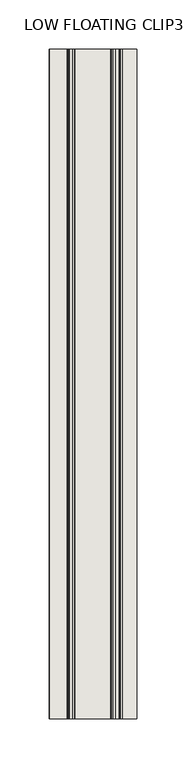
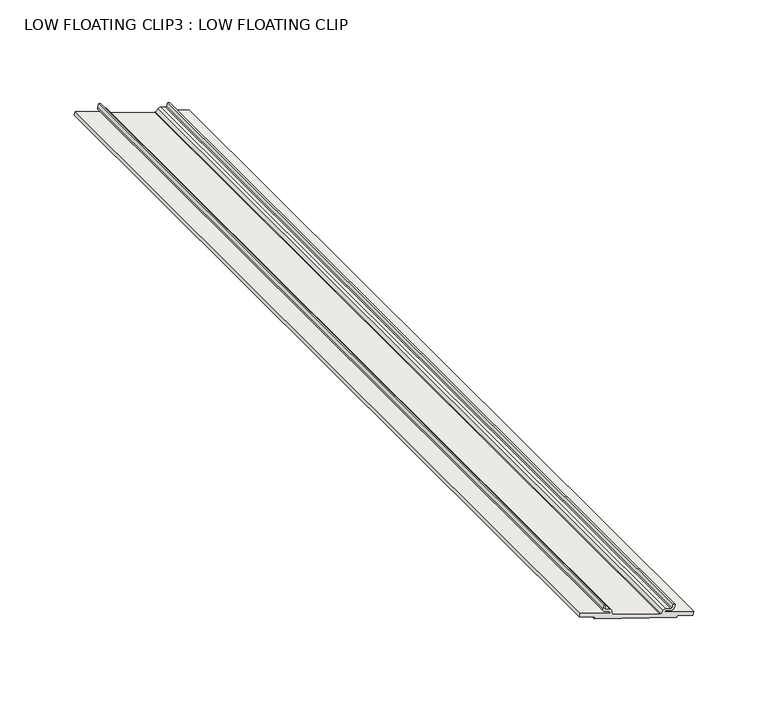
"""IFC4 building model written with IfcOpenShell, lengths in millimetres: wall geometry, LOW FLOATING CLIP3 : LOW FLOATING CLIP."""

from ifc_helpers import new_model, si_unit, frame, origin, place, context, project, spatial, polyline, circle_curve, source, transform, mapped, element, save
from ifc_brep_helpers import plane_surface, cylinder_surface, revolved_surface, advanced_brep


def low_floating_clip3_low_floating_clip_5b88b04a(model_context):
    return source(origin(), model_context, "Body", "AdvancedBrep", [
        advanced_brep(
        [(21637.777683, -2319.6634634, 5817.03297), (21636.9713033, -2319.6634634, 5814.6243705), (21638.3489412, -2319.6634634, 5811.8600323), (21642.3871389, -2319.6634634, 5810.5080761), (21642.464903, -2319.6634634, 5809.3933561), (21619.3927783, -2319.6634634, 5817.117718), (21618.4780847, -2319.6634634, 5814.3855926), (21630.5219314, -2319.6634634, 5810.3534096), (21630.0377864, -2319.6634634, 5808.9073026), (21694.467015, -2319.6634634, 5787.336915), (21694.9511599, -2319.6634634, 5788.7830219), (21706.9950066, -2319.6634634, 5784.7508388), (21707.9097002, -2319.6634634, 5787.4829643), (21684.8375755, -2319.6634634, 5795.2073261), (21685.5708342, -2319.6634634, 5796.0505222), (21689.6090319, -2319.6634634, 5794.6985661), (21692.3733701, -2319.6634634, 5796.076204), (21693.1797499, -2319.6634634, 5798.4848035), (21691.7351297, -2319.6634634, 5798.9684507), (21690.9287499, -2319.6634634, 5796.5598512), (21690.0916213, -2319.6634634, 5796.1431143), (21686.4716883, -2319.6634634, 5797.3550388), (21684.1286763, -2319.6634634, 5796.7167113), (21682.3072646, -2319.6634634, 5794.6221844), (21681.2841484, -2319.6634634, 5794.9647155), (21645.1559643, -2319.6634634, 5807.060141), (21644.1328482, -2319.6634634, 5807.4026721), (21643.9397012, -2319.6634634, 5810.171657), (21642.4533228, -2319.6634634, 5812.0920337), (21638.8333897, -2319.6634634, 5813.3039581), (21638.416463, -2319.6634634, 5814.1405426), (21639.2223032, -2319.6634634, 5816.5493228), (21637.777683, -1637.0384634, 5817.03297), (21639.2223032, -1637.0384634, 5816.5493228), (21638.4159235, -1637.0384634, 5814.1407232), (21638.8333897, -1637.0384634, 5813.3039581), (21642.4533228, -1637.0384634, 5812.0920337), (21643.9397012, -1637.0384634, 5810.171657), (21644.1328482, -1637.0384634, 5807.4026721), (21645.1559643, -1637.0384634, 5807.060141), (21681.2841484, -1637.0384634, 5794.9647155), (21682.3072646, -1637.0384634, 5794.6221844), (21684.1286763, -1637.0384634, 5796.7167113), (21686.4716883, -1637.0384634, 5797.3550388), (21690.0916213, -1637.0384634, 5796.1431143), (21690.9282104, -1637.0384634, 5796.5600318), (21691.7351297, -1637.0384634, 5798.9684507), (21693.1797499, -1637.0384634, 5798.4848035), (21692.3733701, -1637.0384634, 5796.076204), (21689.6090319, -1637.0384634, 5794.6985661), (21685.5708342, -1637.0384634, 5796.0505222), (21684.8375755, -1637.0384634, 5795.2073261), (21707.9097002, -1637.0384634, 5787.4829643), (21706.9950066, -1637.0384634, 5784.7508388), (21694.9511599, -1637.0384634, 5788.7830219), (21694.467015, -1637.0384634, 5787.336915), (21630.0377864, -1637.0384634, 5808.9073026), (21630.5219314, -1637.0384634, 5810.3534096), (21618.4780847, -1637.0384634, 5814.3855926), (21619.3927783, -1637.0384634, 5817.117718), (21642.464903, -1637.0384634, 5809.3933561), (21642.3871389, -1637.0384634, 5810.5080761), (21638.3489412, -1637.0384634, 5811.8600323), (21636.9713033, -1637.0384634, 5814.6243705)],
        [
            (0, 1),
            (1, 2, circle_curve(frame((21639.0422913, -2319.6634634, 5813.9310203), z_axis=(0.0, -1.0, 0.0), x_axis=(-0.9482675310001005, 0.0, 0.31747234470261126)), 2.1839702)),
            (2, 3),
            (3, 4),
            (4, 5),
            (5, 6),
            (6, 7),
            (7, 8),
            (8, 9),
            (9, 10),
            (10, 11),
            (11, 12),
            (12, 13),
            (13, 14),
            (14, 15),
            (15, 16, circle_curve(frame((21690.3023821, -2319.6634634, 5796.7695541), z_axis=(0.0, -1.0, 0.0), x_axis=(0.9482675310000763, 0.0, -0.3174723447026833)), 2.1839702)),
            (16, 17),
            (17, 18),
            (18, 19),
            (19, 20, circle_curve(frame((21690.3014548, -2319.6634634, 5796.7698722), z_axis=(0.0, 1.0, 0.0), x_axis=(-0.3174723447027873, 0.0, -0.9482675310000416)), 0.6609505)),
            (20, 21),
            (21, 22, circle_curve(frame((21685.777847, -2319.6634634, 5795.2825837), z_axis=(0.0, -1.0, 0.0), x_axis=(-0.7545905437642736, 0.0, 0.6561959396868727)), 2.1855173)),
            (22, 23),
            (23, 24),
            (24, 25),
            (25, 26),
            (26, 27),
            (27, 28, circle_curve(frame((21641.7594815, -2319.6634634, 5810.0195786), z_axis=(0.0, -1.0, 0.0), x_axis=(0.997576050299932, 0.0, 0.06958465253191609)), 2.1855173)),
            (28, 29),
            (29, 30, circle_curve(frame((21639.0432232, -2319.6634634, 5813.930716), z_axis=(0.0, 1.0, 0.0), x_axis=(-0.31747234470250746, 0.0, -0.9482675310001353)), 0.6609505)),
            (30, 31),
            (31, 0),
            (32, 33),
            (33, 34),
            (34, 35, circle_curve(frame((21639.0432232, -1637.0384634, 5813.930716), z_axis=(0.0, -1.0, 0.0), x_axis=(-0.31747234470250746, 0.0, -0.9482675310001353)), 0.6609505)),
            (35, 36),
            (36, 37, circle_curve(frame((21641.7594815, -1637.0384634, 5810.0195786), z_axis=(0.0, 1.0, 0.0), x_axis=(0.997576050299932, 0.0, 0.06958465253191609)), 2.1855173)),
            (37, 38),
            (38, 39),
            (39, 40),
            (40, 41),
            (41, 42),
            (42, 43, circle_curve(frame((21685.777847, -1637.0384634, 5795.2825837), z_axis=(0.0, 1.0, 0.0), x_axis=(-0.7545905437642736, 0.0, 0.6561959396868727)), 2.1855173)),
            (43, 44),
            (44, 45, circle_curve(frame((21690.3014548, -1637.0384634, 5796.7698722), z_axis=(0.0, -1.0, 0.0), x_axis=(-0.3174723447027873, 0.0, -0.9482675310000416)), 0.6609505)),
            (45, 46),
            (46, 47),
            (47, 48),
            (48, 49, circle_curve(frame((21690.3023821, -1637.0384634, 5796.7695541), z_axis=(0.0, 1.0, 0.0), x_axis=(0.9482675310000763, 0.0, -0.3174723447026833)), 2.1839702)),
            (49, 50),
            (50, 51),
            (51, 52),
            (52, 53),
            (53, 54),
            (54, 55),
            (55, 56),
            (56, 57),
            (57, 58),
            (58, 59),
            (59, 60),
            (60, 61),
            (61, 62),
            (62, 63, circle_curve(frame((21639.0422913, -1637.0384634, 5813.9310203), z_axis=(0.0, 1.0, 0.0), x_axis=(-0.9482675310001005, 0.0, 0.31747234470261126)), 2.1839702)),
            (63, 32),
            (0, 32),
            (63, 1),
            (62, 2),
            (61, 3),
            (60, 4),
            (59, 5),
            (58, 6),
            (57, 7),
            (56, 8),
            (55, 9),
            (54, 10),
            (53, 11),
            (52, 12),
            (51, 13),
            (50, 14),
            (49, 15),
            (48, 16),
            (47, 17),
            (46, 18),
            (45, 19),
            (44, 20),
            (43, 21),
            (42, 22),
            (41, 23),
            (40, 24),
            (39, 25),
            (38, 26),
            (37, 27),
            (36, 28),
            (35, 29),
            (34, 30),
            (33, 31),
        ],
        [
            plane_surface(frame((21637.777683, -2319.6634634, 5817.03297), z_axis=(0.0, -1.0, 0.0), x_axis=(-0.3174723447025162, 0.0, -0.9482675310001323))),
            plane_surface(frame((21637.777683, -1637.0384634, 5817.03297), z_axis=(0.0, 1.0, 0.0), x_axis=(0.3174723447025162, 0.0, 0.9482675310001323))),
            plane_surface(frame((21637.777683, -2319.6634634, 5817.03297), z_axis=(-0.9482675310001323, 0.0, 0.3174723447025162), x_axis=(0.0, 1.0, 0.0))),
            cylinder_surface(frame((21639.0422913, -1637.0384634, 5813.9310203), z_axis=(0.0, -1.0000000000000002, 0.0), x_axis=(-0.9482675310001005, 0.0, 0.31747234470261126)), 2.1839702),
            plane_surface(frame((21638.3489412, -2319.6634634, 5811.8600323), z_axis=(-0.3174723445422707, 0.0, -0.9482675310537811), x_axis=(0.0, 1.0, 0.0))),
            plane_surface(frame((21642.3871389, -2319.6634634, 5810.5080761), z_axis=(-0.9975755390756385, 0.0, -0.06959198113252213), x_axis=(0.0, 1.0, 0.0))),
            plane_surface(frame((21642.464903, -2319.6634634, 5809.3933561), z_axis=(0.3174723447025733, 0.0, 0.9482675310001131), x_axis=(0.0, 1.0, 0.0))),
            plane_surface(frame((21619.3927783, -2319.6634634, 5817.117718), z_axis=(-0.9482675310001432, 0.0, 0.3174723447024835), x_axis=(0.0, 1.0, 0.0))),
            plane_surface(frame((21618.4780847, -2319.6634634, 5814.3855926), z_axis=(-0.3174723447026279, 0.0, -0.9482675310000949), x_axis=(0.0, 1.0, 0.0))),
            plane_surface(frame((21630.5219314, -2319.6634634, 5810.3534096), z_axis=(-0.9482675310001084, 0.0, 0.31747234470258734), x_axis=(0.0, 1.0, 0.0))),
            plane_surface(frame((21630.0377864, -2319.6634634, 5808.9073026), z_axis=(-0.31747234470254, 0.0, -0.9482675310001243), x_axis=(0.0, 1.0, 0.0))),
            plane_surface(frame((21694.467015, -2319.6634634, 5787.336915), z_axis=(0.9482675310005341, 0.0, -0.3174723447013159), x_axis=(0.0, 1.0, 0.0))),
            plane_surface(frame((21694.9511599, -2319.6634634, 5788.7830219), z_axis=(-0.3174723447026786, 0.0, -0.9482675310000779), x_axis=(0.0, 1.0, 0.0))),
            plane_surface(frame((21706.9950066, -2319.6634634, 5784.7508388), z_axis=(0.9482675310000674, 0.0, -0.31747234470270974), x_axis=(0.0, 1.0, 0.0))),
            plane_surface(frame((21707.9097002, -2319.6634634, 5787.4829643), z_axis=(0.31747234470271984, 0.0, 0.9482675310000641), x_axis=(0.0, 1.0, 0.0))),
            plane_surface(frame((21684.8375755, -2319.6634634, 5795.2073261), z_axis=(0.7545857230581579, 0.0, -0.6562014832022228), x_axis=(0.0, 1.0, 0.0))),
            plane_surface(frame((21685.5708342, -2319.6634634, 5796.0505222), z_axis=(-0.3174723447025522, 0.0, -0.9482675310001202), x_axis=(0.0, 1.0, 0.0))),
            cylinder_surface(frame((21690.3023821, -1637.0384634, 5796.7695541), z_axis=(0.0, -1.0, 0.0), x_axis=(0.9482675310000763, 0.0, -0.3174723447026833)), 2.1839702),
            plane_surface(frame((21692.3733701, -2319.6634634, 5796.076204), z_axis=(0.9482675309984633, 0.0, -0.31747234470750146), x_axis=(0.0, 1.0, 0.0))),
            plane_surface(frame((21693.1797499, -2319.6634634, 5798.4848035), z_axis=(0.3174723447029016, 0.0, 0.9482675310000033), x_axis=(0.0, 1.0, 0.0))),
            plane_surface(frame((21691.7351297, -2319.6634634, 5798.9684507), z_axis=(-0.9482675310001752, 0.0, 0.31747234470238783), x_axis=(0.0, 1.0, 0.0))),
            revolved_surface(polyline([(21690.091621295032, -1637.0384634, 5796.143114301251), (21690.091621295032, -2319.6634634, 5796.143114301251)]), (21690.3014548, -1637.0384634, 5796.7698722), (0.0, 1.0000000000000002, 0.0)),
            plane_surface(frame((21690.0916213, -2319.6634634, 5796.1431143), z_axis=(0.31747234470292157, 0.0, 0.9482675309999966), x_axis=(0.0, 1.0, 0.0))),
            cylinder_surface(frame((21685.777847, -1637.0384634, 5795.2825837), z_axis=(0.0, -1.0000000000000002, 0.0), x_axis=(-0.7545905437642736, 0.0, 0.6561959396868727)), 2.1855173),
            plane_surface(frame((21684.1286763, -2319.6634634, 5796.7167113), z_axis=(-0.7545905437681126, 0.0, 0.656195939682458), x_axis=(0.0, 1.0, 0.0))),
            plane_surface(frame((21682.3072646, -2319.6634634, 5794.6221844), z_axis=(0.31747234470267577, 0.0, 0.9482675310000789), x_axis=(0.0, 1.0, 0.0))),
            plane_surface(frame((21681.2841484, -2319.6634634, 5794.9647155), z_axis=(0.3174723447026769, 0.0, 0.9482675310000784), x_axis=(0.0, 1.0, 0.0))),
            plane_surface(frame((21645.1559643, -2319.6634634, 5807.060141), z_axis=(0.31747234470207936, 0.0, 0.9482675310002785), x_axis=(0.0, 1.0, 0.0))),
            plane_surface(frame((21644.1328482, -2319.6634634, 5807.4026721), z_axis=(0.9975760502999373, 0.0, 0.06958465253183929), x_axis=(0.0, 1.0, 0.0))),
            cylinder_surface(frame((21641.7594815, -1637.0384634, 5810.0195786), z_axis=(0.0, -1.0, 0.0), x_axis=(0.997576050299932, 0.0, 0.06958465253191609)), 2.1855173),
            plane_surface(frame((21642.4533228, -2319.6634634, 5812.0920337), z_axis=(0.317472342372389, 0.0, 0.9482675317802401), x_axis=(0.0, 1.0, 0.0))),
            revolved_surface(polyline([(21638.83338969503, -1637.0384634, 5813.303958101252), (21638.83338969503, -2319.6634634, 5813.303958101252)]), (21639.0432232, -1637.0384634, 5813.930716), (0.0, 1.0000000000000002, 0.0)),
            plane_surface(frame((21638.4159235, -2319.6634634, 5814.1407232), z_axis=(0.9482675310001136, 0.0, -0.3174723447025722), x_axis=(0.0, 1.0, 0.0))),
            plane_surface(frame((21639.2223032, -2319.6634634, 5816.5493228), z_axis=(0.3174723447026848, 0.0, 0.9482675310000759), x_axis=(0.0, 1.0, 0.0))),
        ],
        [
            (0, [[1, 2, 3, 4, 5, 6, 7, 8, 9, 10, 11, 12, 13, 14, 15, 16, 17, 18, 19, 20, 21, 22, 23, 24, 25, 26, 27, 28, 29, 30, 31, 32]]),
            (1, [[33, 34, 35, 36, 37, 38, 39, 40, 41, 42, 43, 44, 45, 46, 47, 48, 49, 50, 51, 52, 53, 54, 55, 56, 57, 58, 59, 60, 61, 62, 63, 64]]),
            (2, [[-1, 65, -64, 66]]),
            (3, [[-2, -66, -63, 67]]),
            (4, [[-3, -67, -62, 68]]),
            (5, [[-4, -68, -61, 69]]),
            (6, [[-5, -69, -60, 70]]),
            (7, [[-6, -70, -59, 71]]),
            (8, [[-7, -71, -58, 72]]),
            (9, [[-8, -72, -57, 73]]),
            (10, [[-9, -73, -56, 74]]),
            (11, [[-10, -74, -55, 75]]),
            (12, [[-11, -75, -54, 76]]),
            (13, [[-12, -76, -53, 77]]),
            (14, [[-13, -77, -52, 78]]),
            (15, [[-14, -78, -51, 79]]),
            (16, [[-15, -79, -50, 80]]),
            (17, [[-16, -80, -49, 81]]),
            (18, [[-17, -81, -48, 82]]),
            (19, [[-18, -82, -47, 83]]),
            (20, [[-19, -83, -46, 84]]),
            (21, [[-20, -84, -45, 85]]),
            (22, [[-21, -85, -44, 86]]),
            (23, [[-22, -86, -43, 87]]),
            (24, [[-23, -87, -42, 88]]),
            (25, [[-24, -88, -41, 89]]),
            (26, [[-25, -89, -40, 90]]),
            (27, [[-26, -90, -39, 91]]),
            (28, [[-27, -91, -38, 92]]),
            (29, [[-28, -92, -37, 93]]),
            (30, [[-29, -93, -36, 94]]),
            (31, [[-30, -94, -35, 95]]),
            (32, [[-31, -95, -34, 96]]),
            (33, [[-32, -96, -33, -65]]),
        ],
    ),
    ])


if __name__ == "__main__":
    model = new_model("IFC4")
    model_context = context("Model", 3, world=origin())
    ifc_project = project(units=[si_unit("LENGTHUNIT", "METRE", prefix="MILLI")], contexts=[model_context])
    site = spatial("IfcSite", under=ifc_project)
    building = spatial("IfcBuilding", under=site)
    placement = place(None, origin())
    low_floating_clip3_low_floating_clip_shape = low_floating_clip3_low_floating_clip_5b88b04a(model_context)
    element("IfcWall", 1, ObjectType="LOW FLOATING CLIP3 : LOW FLOATING CLIP", at=placement, inside=building, context=model_context, shape_type="MappedRepresentation", body=[
        mapped(low_floating_clip3_low_floating_clip_shape, transform((0.0, 0.0, 0.0), x_axis=(1.0, 0.0, 0.0), y_axis=(0.0, 1.0, 0.0), z_axis=(0.0, 0.0, 1.0))),
    ])
    save(model, "model.ifc")

# Revit data of these elements
# Element 1 (IfcWall, "LOW FLOATING CLIP3 : LOW FLOATING CLIP")
#   Materials on its faces: "LOW FLOATING CLIP"
# Materials
#   "LOW FLOATING CLIP": class "Metal", colour RGB 247 247 247, transparency 0, Cost = 0
